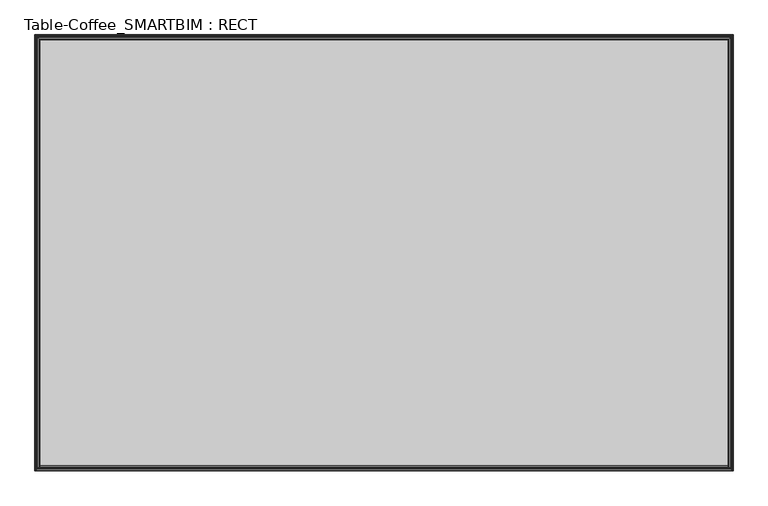
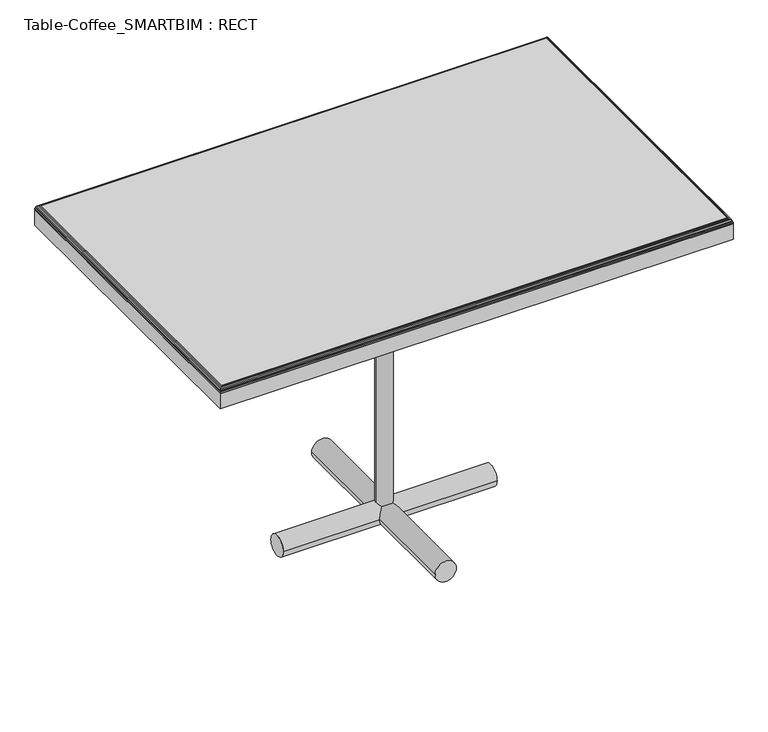
"""IFC4 building model written with IfcOpenShell, lengths in millimetres: furniture geometry, Table-Coffee_SMARTBIM : RECT."""

import ifcopenshell
import ifcopenshell.guid

model = None  # the IFC model being written
_history = None  # IfcOwnerHistory: only IFC2X3 demands one
_inside = {}  # id of a spatial element -> (the spatial element, [elements in it])
_under = {}  # id of a project, library or spatial element -> (it, [spatial elements below it])
_declared = {}  # id of a project -> (the project, [libraries it declares])
_typed = {}  # id of a type object -> (the type object, [elements of that type])
_made_of = {}  # id of a material, layer set ... -> (it, [elements and type objects made of it])


def new_model(schema):
    """Start an empty IFC model of exactly this schema.

    Asked for "IFC4X3", IfcOpenShell would pick the latest addendum, in which some entities
    have other attributes; the version numbers below select the first issue.
    IFC2X3 requires an IfcOwnerHistory on every rooted entity: one is made here for all.
    """
    global model, _history
    if schema == "IFC4X3":
        model = ifcopenshell.file(schema_version=(4, 3, 0, 0))
    else:
        model = ifcopenshell.file(schema=schema)
    _inside.clear()
    _under.clear()
    _declared.clear()
    _typed.clear()
    _made_of.clear()
    _history = None
    if model.schema == "IFC2X3":
        org = make("IfcOrganization", Name="unknown")
        user = make(
            "IfcPersonAndOrganization",
            ThePerson=make("IfcPerson", FamilyName="unknown"),
            TheOrganization=org,
        )
        app = make(
            "IfcApplication",
            ApplicationDeveloper=org,
            Version="unknown",
            ApplicationFullName="unknown",
            ApplicationIdentifier="unknown",
        )
        _history = make(
            "IfcOwnerHistory",
            OwningUser=user,
            OwningApplication=app,
            ChangeAction="ADDED",
            CreationDate=0,
        )
    return model


def make(cls, **values):
    """One entity of the class cls with the attributes given. An attribute that is None is left unset."""
    return model.create_entity(
        cls, **{name: value for name, value in values.items() if value is not None}
    )


def rooted(cls, **values):
    """An entity with a GlobalId (a new one), such as an element, a storey or a relation."""
    return make(cls, GlobalId=ifcopenshell.guid.new(), OwnerHistory=_history, **values)


def si_unit(unit_type, name, prefix=None):
    """IfcSIUnit, for example si_unit("LENGTHUNIT", "METRE", prefix="MILLI")."""
    return make("IfcSIUnit", UnitType=unit_type, Prefix=prefix, Name=name)


def assignment(units):
    """IfcUnitAssignment: the units of a project."""
    return None if units is None else make("IfcUnitAssignment", Units=units)


def point(xyz):
    """IfcCartesianPoint."""
    return None if xyz is None else make("IfcCartesianPoint", Coordinates=xyz)


def direction(xyz):
    """IfcDirection."""
    return None if xyz is None else make("IfcDirection", DirectionRatios=xyz)


def frame(location, z_axis=None, x_axis=None):
    """IfcAxis2Placement3D, a coordinate frame: its origin and axes. An axis left out is left unset."""
    return make(
        "IfcAxis2Placement3D",
        Location=point(location),
        Axis=direction(z_axis),
        RefDirection=direction(x_axis),
    )


def frame_2d(location, x_axis=None):
    """IfcAxis2Placement2D, a coordinate frame in the plane: its origin and x axis."""
    return make(
        "IfcAxis2Placement2D", Location=point(location), RefDirection=direction(x_axis)
    )


def origin():
    """The frame at (0, 0, 0) with its axes left unset."""
    return frame((0.0, 0.0, 0.0))


def origin_2d():
    """The frame at (0, 0) in the plane with its x axis left unset."""
    return frame_2d((0.0, 0.0))


def place(relative_to, where):
    """IfcLocalPlacement: puts the frame where relative to a parent placement (None: the world)."""
    return make(
        "IfcLocalPlacement", PlacementRelTo=relative_to, RelativePlacement=where
    )


def context(
    kind, dimensions, precision=None, world=None, true_north=None, identifier=None
):
    """IfcGeometricRepresentationContext, for example the 3D "Model" context."""
    return make(
        "IfcGeometricRepresentationContext",
        ContextIdentifier=identifier,
        ContextType=kind,
        CoordinateSpaceDimension=dimensions,
        Precision=precision,
        WorldCoordinateSystem=world,
        TrueNorth=true_north,
    )


def project(units=None, contexts=None):
    """IfcProject with its units and contexts."""
    return rooted(
        "IfcProject",
        Name="project",
        RepresentationContexts=contexts,
        UnitsInContext=assignment(units),
    )


def spatial(cls, under=None, at=None, **own):
    """A site, building, storey or space (cls), placed at a placement, below another one or the project."""
    s = rooted(cls, ObjectPlacement=at, **own)
    if under is not None:
        _under.setdefault(under.id(), (under, []))[1].append(s)
    return s


def polyline(points):
    """IfcPolyline through the points."""
    return make("IfcPolyline", Points=[point(p) for p in points])


def circle_curve(where, radius):
    """IfcCircle in the frame where."""
    return make("IfcCircle", Position=where, Radius=radius)


def ellipse_curve(where, semi_axis1, semi_axis2):
    """IfcEllipse in the frame where."""
    return make(
        "IfcEllipse", Position=where, SemiAxis1=semi_axis1, SemiAxis2=semi_axis2
    )


def trimmed(basis, trim1, trim2, sense, master):
    """IfcTrimmedCurve: the piece of a basis curve between two trims."""
    return make(
        "IfcTrimmedCurve",
        BasisCurve=basis,
        Trim1=trim1,
        Trim2=trim2,
        SenseAgreement=sense,
        MasterRepresentation=master,
    )


def segment(curve, same_sense, transition):
    """IfcCompositeCurveSegment."""
    return make(
        "IfcCompositeCurveSegment",
        Transition=transition,
        SameSense=same_sense,
        ParentCurve=curve,
    )


def composite_curve(segments, self_intersect=None):
    """IfcCompositeCurve: segments joined end to end."""
    return make("IfcCompositeCurve", Segments=segments, SelfIntersect=self_intersect)


def outline(outer, holes=None, kind="AREA"):
    """IfcArbitraryClosedProfileDef: a profile drawn as a closed curve; with holes, ...WithVoids."""
    if holes is None:
        return make("IfcArbitraryClosedProfileDef", ProfileType=kind, OuterCurve=outer)
    return make(
        "IfcArbitraryProfileDefWithVoids",
        ProfileType=kind,
        OuterCurve=outer,
        InnerCurves=holes,
    )


def extrude(swept, where, along, depth):
    """IfcExtrudedAreaSolid: the profile swept, set in the frame where, extruded along a direction by depth."""
    return make(
        "IfcExtrudedAreaSolid",
        SweptArea=swept,
        Position=where,
        ExtrudedDirection=direction(along),
        Depth=depth,
    )


def shape(context_of_items, identifier, shape_type, items):
    """IfcShapeRepresentation: the items that make up one representation, for example the "Body"."""
    return make(
        "IfcShapeRepresentation",
        ContextOfItems=context_of_items,
        RepresentationIdentifier=identifier,
        RepresentationType=shape_type,
        Items=items,
    )


def source(mapping_origin, context_of_items, identifier, shape_type, items):
    """IfcRepresentationMap: a shape defined once, which mapped items show again and again."""
    return make(
        "IfcRepresentationMap",
        MappingOrigin=mapping_origin,
        MappedRepresentation=shape(context_of_items, identifier, shape_type, items),
    )


def transform(
    local_origin,
    x_axis=None,
    y_axis=None,
    z_axis=None,
    scale=None,
    scale2=None,
    scale3=None,
    uniform=True,
):
    """IfcCartesianTransformationOperator3D, or its non-uniform kind. x_axis, y_axis, z_axis: its Axis1, 2, 3."""
    if uniform:
        return make(
            "IfcCartesianTransformationOperator3D",
            Axis1=direction(x_axis),
            Axis2=direction(y_axis),
            LocalOrigin=point(local_origin),
            Scale=scale,
            Axis3=direction(z_axis),
        )
    return make(
        "IfcCartesianTransformationOperator3DnonUniform",
        Axis1=direction(x_axis),
        Axis2=direction(y_axis),
        LocalOrigin=point(local_origin),
        Scale=scale,
        Axis3=direction(z_axis),
        Scale2=scale2,
        Scale3=scale3,
    )


def mapped(mapping_source, mapping_target):
    """IfcMappedItem: shows the shape of a source again, moved by a transform."""
    return make(
        "IfcMappedItem", MappingSource=mapping_source, MappingTarget=mapping_target
    )


def made_of(thing, what):
    """Note that an element or type object is made of a material, layer set ...; save() writes the relation."""
    if what is not None:
        _made_of.setdefault(what.id(), (what, []))[1].append(thing)
    return thing


def element(
    cls,
    number,
    at=None,
    inside=None,
    cuts=None,
    type_object=None,
    material=None,
    context=None,
    identifier="Body",
    shape_type=None,
    held_by="IfcProductDefinitionShape",
    body=None,
    shapes=None,
    **own,
):
    """One element of the class cls, such as IfcWall. Its Tag is "e" and its number.

    at: its placement. inside: the storey or other place that contains it. cuts: it is an
    opening in that element (IfcRelVoidsElement). A single representation is given by context,
    identifier, shape_type and body (its items); several are given by shapes. held_by: the class
    of the entity that holds the representations. save() writes the other relations.
    """
    e = rooted(cls, Tag="e%d" % number, ObjectPlacement=at, **own)
    if body is not None:
        shapes = [shape(context, identifier, shape_type, body)]
    if shapes is not None:
        e.Representation = make(held_by, Representations=shapes)
    if inside is not None:
        _inside.setdefault(inside.id(), (inside, []))[1].append(e)
    if cuts is not None:
        rooted(
            "IfcRelVoidsElement", RelatingBuildingElement=cuts, RelatedOpeningElement=e
        )
    if type_object is not None:
        _typed.setdefault(type_object.id(), (type_object, []))[1].append(e)
    return made_of(e, material)


def aggregate(whole, parts):
    """IfcRelAggregates: a whole, such as a stair, and the parts it consists of."""
    return rooted("IfcRelAggregates", RelatingObject=whole, RelatedObjects=parts)


def save(model, path):
    """Write the relations noted so far, then the file.

    IfcRelAggregates (storeys below a building ...), IfcRelContainedInSpatialStructure (elements
    in a storey), IfcRelDefinesByType, IfcRelAssociatesMaterial and IfcRelDeclares: one each for
    every whole, place, type object, material and project.
    """
    for whole, parts in _under.values():
        aggregate(whole, parts)
    for where, things in _inside.values():
        rooted(
            "IfcRelContainedInSpatialStructure",
            RelatedElements=things,
            RelatingStructure=where,
        )
    for kind, things in _typed.values():
        rooted("IfcRelDefinesByType", RelatedObjects=things, RelatingType=kind)
    for what, things in _made_of.values():
        rooted("IfcRelAssociatesMaterial", RelatedObjects=things, RelatingMaterial=what)
    for by, libraries in _declared.values():
        rooted("IfcRelDeclares", RelatingContext=by, RelatedDefinitions=libraries)
    model.write(path)


def plane_surface(at):
    """IfcPlane: the flat surface through the origin of the frame at, square to its z axis."""
    return make("IfcPlane", Position=at)


def cylinder_surface(at, radius):
    """IfcCylindricalSurface: all points at the distance radius from the z axis of the frame at."""
    return make("IfcCylindricalSurface", Position=at, Radius=radius)


def advanced_brep(points, edges, surfaces, faces):
    """IfcAdvancedBrep: a solid bounded by faces that lie on surfaces and meet in shared edges.

    An edge is (start, end): straight between two places in points (the first is 0);
    or (start, end, curve); or (start, end, curve, False) where it runs against its curve.
    A face is (place in surfaces, loops), or (place, loops, False) where it looks against
    its surface's normal. A loop lists edges by number (the first is 1), with a minus sign
    where the edge is run from its end to its start. The first loop is the outer one.
    """
    corners = [point(p) for p in points]
    vertices = [make("IfcVertexPoint", VertexGeometry=c) for c in corners]
    made = []
    for start, end, *more in edges:
        made.append(
            make(
                "IfcEdgeCurve",
                EdgeStart=vertices[start],
                EdgeEnd=vertices[end],
                EdgeGeometry=more[0] if more else make("IfcPolyline", Points=[corners[start], corners[end]]),
                SameSense=more[1] if len(more) > 1 else True,
            )
        )
    hull = []
    for where, loops, *sense in faces:
        bounds = []
        for j, loop in enumerate(loops):
            ring = [make("IfcOrientedEdge", EdgeElement=made[abs(k) - 1], Orientation=k > 0) for k in loop]
            bounds.append(
                make(
                    "IfcFaceOuterBound" if j == 0 else "IfcFaceBound",
                    Bound=make("IfcEdgeLoop", EdgeList=ring),
                    Orientation=True,
                )
            )
        hull.append(make("IfcAdvancedFace", Bounds=bounds, FaceSurface=surfaces[where], SameSense=sense[0] if sense else True))
    return make("IfcAdvancedBrep", Outer=make("IfcClosedShell", CfsFaces=hull))


def table_coffee_smartbim_rect_06f34b69(model_context):
    return source(origin(), model_context, "Body", "SolidModel", [
        extrude(outline(composite_curve([segment(trimmed(circle_curve(frame_2d((0.0, 25.4)), 25.4), [point((-25.4, 25.4))], [point((25.4, 25.4))], False, "CARTESIAN"), True, "CONTINUOUS"), segment(trimmed(circle_curve(frame_2d((0.0, 25.4)), 25.4), [point((25.4, 25.4))], [point((-25.4, 25.4))], False, "CARTESIAN"), True, "CONTINUOUS")], self_intersect=False)), frame((-254.0, 0.0, 0.0), z_axis=(1.0, 0.0, 0.0), x_axis=(0.0, 1.0, 0.0)), (0.0, 0.0, 1.0), 508.0),
        extrude(outline(composite_curve([segment(trimmed(circle_curve(frame_2d((25.4, 0.0)), 25.4), [point((25.4, -25.4))], [point((25.4, 25.4))], False, "CARTESIAN"), True, "CONTINUOUS"), segment(trimmed(circle_curve(frame_2d((25.4, 0.0)), 25.4), [point((25.4, 25.4))], [point((25.4, -25.4))], False, "CARTESIAN"), True, "CONTINUOUS")], self_intersect=False)), frame((0.0, -254.0, 0.0), z_axis=(0.0, 1.0, 0.0), x_axis=(0.0, 0.0, 1.0)), (0.0, 0.0, 1.0), 508.0),
        extrude(outline(polyline([(609.6, -381.0), (-609.6, -381.0), (-609.6, 381.0), (609.6, 381.0), (609.6, -381.0)])), frame((0.0, 0.0, 723.9), z_axis=(0.0, 0.0, 1.0), x_axis=(1.0, 0.0, 0.0)), (0.0, 0.0, 1.0), 38.1),
        advanced_brep(
        [(-600.1998654, 371.5998654, 774.7), (-600.1998654, -371.5998654, 774.7), (600.1998654, -371.5998654, 774.7), (600.1998654, 371.5998654, 774.7), (609.6, -381.0, 762.0), (-609.6, -381.0, 762.0), (-609.6, 381.0, 762.0), (609.6, 381.0, 762.0), (609.6, -381.0, 765.2998654), (-609.6, -381.0, 765.2998654), (-609.6, 381.0, 765.2998654), (609.6, 381.0, 765.2998654), (-609.2372483, -380.6372483, 767.8860287), (-609.2372483, 380.6372483, 767.8860287), (-602.3616212, -373.7616212, 774.4480533), (-602.3616212, 373.7616212, 774.4480533), (-604.3639185, 375.7639185, 773.7273912), (-604.3639185, -375.7639185, 773.7273912), (-606.4885738, 377.8885738, 772.2866155), (-606.4885738, -377.8885738, 772.2866155), (-608.5102962, 379.9102962, 769.692959), (-608.5102962, -379.9102962, 769.692959), (609.2372483, 380.6372483, 767.8860287), (602.3616212, 373.7616212, 774.4480533), (604.3639185, 375.7639185, 773.7273912), (606.4885738, 377.8885738, 772.2866155), (608.5102962, 379.9102962, 769.692959), (609.2372483, -380.6372483, 767.8860287), (602.3616212, -373.7616212, 774.4480533), (604.3639185, -375.7639185, 773.7273912), (606.4885738, -377.8885738, 772.2866155), (608.5102962, -379.9102962, 769.692959)],
        [
            (0, 1),
            (1, 2),
            (2, 3),
            (3, 0),
            (4, 5),
            (5, 6),
            (6, 7),
            (7, 4),
            (4, 8),
            (8, 9),
            (9, 5),
            (9, 10),
            (10, 6),
            (10, 11),
            (11, 7),
            (11, 8),
            (9, 12, ellipse_curve(frame((-600.1998654, -371.5998654, 765.2998654), z_axis=(-0.7071067811865475, 0.7071067811865475, 0.0), x_axis=(0.7071067811865474, 0.7071067811865476, 0.0)), 13.2937978, 9.4001346)),
            (12, 13),
            (13, 10, ellipse_curve(frame((-600.1998654, 371.5998654, 765.2998654), z_axis=(-0.7071067811865475, -0.7071067811865475, 0.0), x_axis=(-0.7071067811865474, 0.7071067811865476, 0.0)), 13.2937978, 9.4001346)),
            (14, 1, ellipse_curve(frame((-600.1998654, -371.5998654, 765.2998654), z_axis=(-0.7071067811865475, 0.7071067811865475, 0.0), x_axis=(0.7071067811865474, 0.7071067811865476, 0.0)), 13.2937978, 9.4001346)),
            (0, 15, ellipse_curve(frame((-600.1998654, 371.5998654, 765.2998654), z_axis=(-0.7071067811865475, -0.7071067811865475, 0.0), x_axis=(-0.7071067811865474, 0.7071067811865476, 0.0)), 13.2937978, 9.4001346)),
            (15, 14),
            (15, 16, ellipse_curve(frame((-600.1998654, 371.5998654, 765.2998654), z_axis=(-0.7071067811865475, -0.7071067811865475, 0.0), x_axis=(-0.7071067811865474, 0.7071067811865476, 0.0)), 13.2937978, 9.4001346)),
            (16, 17),
            (17, 14, ellipse_curve(frame((-600.1998654, -371.5998654, 765.2998654), z_axis=(-0.7071067811865475, 0.7071067811865475, 0.0), x_axis=(0.7071067811865474, 0.7071067811865476, 0.0)), 13.2937978, 9.4001346)),
            (16, 18, ellipse_curve(frame((-600.1998654, 371.5998654, 765.2998654), z_axis=(-0.7071067811865475, -0.7071067811865475, 0.0), x_axis=(-0.7071067811865474, 0.7071067811865476, 0.0)), 13.2937978, 9.4001346)),
            (18, 19),
            (19, 17, ellipse_curve(frame((-600.1998654, -371.5998654, 765.2998654), z_axis=(-0.7071067811865475, 0.7071067811865475, 0.0), x_axis=(0.7071067811865474, 0.7071067811865476, 0.0)), 13.2937978, 9.4001346)),
            (18, 20, ellipse_curve(frame((-600.1998654, 371.5998654, 765.2998654), z_axis=(-0.7071067811865475, -0.7071067811865475, 0.0), x_axis=(-0.7071067811865474, 0.7071067811865476, 0.0)), 13.2937978, 9.4001346)),
            (20, 21),
            (21, 19, ellipse_curve(frame((-600.1998654, -371.5998654, 765.2998654), z_axis=(-0.7071067811865475, 0.7071067811865475, 0.0), x_axis=(0.7071067811865474, 0.7071067811865476, 0.0)), 13.2937978, 9.4001346)),
            (12, 21, ellipse_curve(frame((-600.1998654, -371.5998654, 765.2998654), z_axis=(-0.7071067811865475, 0.7071067811865475, 0.0), x_axis=(0.7071067811865474, 0.7071067811865476, 0.0)), 13.2937978, 9.4001346)),
            (20, 13, ellipse_curve(frame((-600.1998654, 371.5998654, 765.2998654), z_axis=(-0.7071067811865475, -0.7071067811865475, 0.0), x_axis=(-0.7071067811865474, 0.7071067811865476, 0.0)), 13.2937978, 9.4001346)),
            (13, 22),
            (22, 11, ellipse_curve(frame((600.1998654, 371.5998654, 765.2998654), z_axis=(-0.7071067811865475, 0.7071067811865475, 0.0), x_axis=(0.7071067811865476, 0.7071067811865474, 0.0)), 13.2937978, 9.4001346)),
            (3, 23, ellipse_curve(frame((600.1998654, 371.5998654, 765.2998654), z_axis=(-0.7071067811865475, 0.7071067811865475, 0.0), x_axis=(0.7071067811865476, 0.7071067811865474, 0.0)), 13.2937978, 9.4001346)),
            (23, 15),
            (23, 24, ellipse_curve(frame((600.1998654, 371.5998654, 765.2998654), z_axis=(-0.7071067811865475, 0.7071067811865475, 0.0), x_axis=(0.7071067811865476, 0.7071067811865474, 0.0)), 13.2937978, 9.4001346)),
            (24, 16),
            (24, 25, ellipse_curve(frame((600.1998654, 371.5998654, 765.2998654), z_axis=(-0.7071067811865475, 0.7071067811865475, 0.0), x_axis=(0.7071067811865476, 0.7071067811865474, 0.0)), 13.2937978, 9.4001346)),
            (25, 18),
            (25, 26, ellipse_curve(frame((600.1998654, 371.5998654, 765.2998654), z_axis=(-0.7071067811865475, 0.7071067811865475, 0.0), x_axis=(0.7071067811865476, 0.7071067811865474, 0.0)), 13.2937978, 9.4001346)),
            (26, 20),
            (26, 22, ellipse_curve(frame((600.1998654, 371.5998654, 765.2998654), z_axis=(-0.7071067811865475, 0.7071067811865475, 0.0), x_axis=(0.7071067811865476, 0.7071067811865474, 0.0)), 13.2937978, 9.4001346)),
            (22, 27),
            (27, 8, ellipse_curve(frame((600.1998654, -371.5998654, 765.2998654), z_axis=(0.7071067811865475, 0.7071067811865475, 0.0), x_axis=(0.7071067811865474, -0.7071067811865476, 0.0)), 13.2937978, 9.4001346)),
            (2, 28, ellipse_curve(frame((600.1998654, -371.5998654, 765.2998654), z_axis=(0.7071067811865475, 0.7071067811865475, 0.0), x_axis=(0.7071067811865474, -0.7071067811865476, 0.0)), 13.2937978, 9.4001346)),
            (28, 23),
            (28, 29, ellipse_curve(frame((600.1998654, -371.5998654, 765.2998654), z_axis=(0.7071067811865475, 0.7071067811865475, 0.0), x_axis=(0.7071067811865474, -0.7071067811865476, 0.0)), 13.2937978, 9.4001346)),
            (29, 24),
            (29, 30, ellipse_curve(frame((600.1998654, -371.5998654, 765.2998654), z_axis=(0.7071067811865475, 0.7071067811865475, 0.0), x_axis=(0.7071067811865474, -0.7071067811865476, 0.0)), 13.2937978, 9.4001346)),
            (30, 25),
            (30, 31, ellipse_curve(frame((600.1998654, -371.5998654, 765.2998654), z_axis=(0.7071067811865475, 0.7071067811865475, 0.0), x_axis=(0.7071067811865474, -0.7071067811865476, 0.0)), 13.2937978, 9.4001346)),
            (31, 26),
            (31, 27, ellipse_curve(frame((600.1998654, -371.5998654, 765.2998654), z_axis=(0.7071067811865475, 0.7071067811865475, 0.0), x_axis=(0.7071067811865474, -0.7071067811865476, 0.0)), 13.2937978, 9.4001346)),
            (27, 12),
            (14, 28),
            (17, 29),
            (19, 30),
            (21, 31),
        ],
        [
            plane_surface(frame((-609.6, -381.0, 774.7), z_axis=(0.0, 0.0, 1.0), x_axis=(-1.0, 0.0, 0.0))),
            plane_surface(frame((-609.6, -381.0, 762.0), z_axis=(0.0, 0.0, -1.0), x_axis=(1.0, 0.0, 0.0))),
            plane_surface(frame((609.6, -381.0, 774.7), z_axis=(0.0, -1.0, 0.0), x_axis=(0.0, 0.0, -1.0))),
            plane_surface(frame((-609.6, -381.0, 774.7), z_axis=(-1.0, 0.0, 0.0), x_axis=(0.0, 0.0, -1.0))),
            plane_surface(frame((-609.6, 381.0, 774.7), z_axis=(0.0, 1.0, 0.0), x_axis=(0.0, 0.0, -1.0))),
            plane_surface(frame((609.6, 381.0, 774.7), z_axis=(1.0, 0.0, 0.0), x_axis=(0.0, 0.0, -1.0))),
            cylinder_surface(frame((-600.1998654, -381.0, 765.2998654), z_axis=(0.0, 1.0, 0.0), x_axis=(1.0, 0.0, 0.0)), 9.4001346),
            cylinder_surface(frame((-609.6, 371.5998654, 765.2998654), z_axis=(1.0, 0.0, 0.0), x_axis=(0.0, -1.0, 0.0)), 9.4001346),
            cylinder_surface(frame((600.1998654, 381.0, 765.2998654), z_axis=(0.0, -1.0, 0.0), x_axis=(-1.0, 0.0, 0.0)), 9.4001346),
            cylinder_surface(frame((609.6, -371.5998654, 765.2998654), z_axis=(-1.0, 0.0, 0.0), x_axis=(0.0, 1.0, 0.0)), 9.4001346),
        ],
        [
            (0, [[1, 2, 3, 4]]),
            (1, [[5, 6, 7, 8]]),
            (2, [[9, 10, 11, -5]]),
            (3, [[-11, 12, 13, -6]]),
            (4, [[-13, 14, 15, -7]]),
            (5, [[-15, 16, -9, -8]]),
            (6, [[-12, 17, 18, 19]]),
            (6, [[20, -1, 21, 22]]),
            (6, [[23, 24, 25, -22]]),
            (6, [[26, 27, 28, -24]]),
            (6, [[29, 30, 31, -27]]),
            (6, [[32, -30, 33, -18]]),
            (7, [[34, 35, -14, -19]]),
            (7, [[-4, 36, 37, -21]]),
            (7, [[-37, 38, 39, -23]]),
            (7, [[-39, 40, 41, -26]]),
            (7, [[-41, 42, 43, -29]]),
            (7, [[-43, 44, -34, -33]]),
            (8, [[45, 46, -16, -35]]),
            (8, [[-3, 47, 48, -36]]),
            (8, [[-48, 49, 50, -38]]),
            (8, [[-50, 51, 52, -40]]),
            (8, [[-52, 53, 54, -42]]),
            (8, [[-54, 55, -45, -44]]),
            (9, [[-10, -46, 56, -17]]),
            (9, [[57, -47, -2, -20]]),
            (9, [[58, -49, -57, -25]]),
            (9, [[59, -51, -58, -28]]),
            (9, [[60, -53, -59, -31]]),
            (9, [[-56, -55, -60, -32]]),
        ],
    ),
        extrude(outline(polyline([(76.2, -76.2), (-76.2, -76.2), (-76.2, 76.2), (76.2, 76.2), (76.2, -76.2)])), frame((0.0, 0.0, 755.65), z_axis=(0.0, 0.0, 1.0), x_axis=(1.0, 0.0, 0.0)), (0.0, 0.0, 1.0), 6.35),
        extrude(outline(composite_curve([segment(trimmed(circle_curve(origin_2d(), 19.05), [point((-19.05, 0.0))], [point((19.05, 0.0))], False, "CARTESIAN"), True, "CONTINUOUS"), segment(trimmed(circle_curve(origin_2d(), 19.05), [point((19.05, 0.0))], [point((-19.05, 0.0))], False, "CARTESIAN"), True, "CONTINUOUS")], self_intersect=False)), frame((0.0, 0.0, 24.2070278), z_axis=(0.0, 0.0, 1.0), x_axis=(1.0, 0.0, 0.0)), (0.0, 0.0, 1.0), 731.4429722),
    ])


if __name__ == "__main__":
    model = new_model("IFC4")
    model_context = context("Model", 3, world=origin())
    ifc_project = project(units=[si_unit("LENGTHUNIT", "METRE", prefix="MILLI")], contexts=[model_context])
    site = spatial("IfcSite", under=ifc_project)
    building = spatial("IfcBuilding", under=site)
    placement = place(None, origin())
    table_coffee_smartbim_rect_shape = table_coffee_smartbim_rect_06f34b69(model_context)
    element("IfcFurniture", 1, ObjectType="Table-Coffee_SMARTBIM : RECT", at=placement, inside=building, context=model_context, shape_type="MappedRepresentation", body=[
        mapped(table_coffee_smartbim_rect_shape, transform((0.0, 0.0, 0.0), x_axis=(1.0, 0.0, 0.0), y_axis=(0.0, 1.0, 0.0), z_axis=(0.0, 0.0, 1.0))),
    ])
    save(model, "model.ifc")

# Revit data of these elements
# Project information
#   Project Issue Date = "08/08/2019"
#   Project Status = "Project Status"
#   Client Name = "Owner"
#   Project Address = "SOMERS, WI"
#   Project Name = "OAKFIRE 2.0"
#   Project Number = "Project Number"
# Type "Table-Coffee_SMARTBIM : RECT"
#   Subcategory = "Table\r\n"
#   SmartBIM Object Created By = "SMARTBIM, LLC"
#   Manufacturer = "SMARTBIM"
#   Assembly Code = "E2020200"
#   95 CSI = "12500"
#   04 CSI = "12 50 00"
#   table cloth = 0' - 1 1/2"
#   Width = 4' - 0"
#   SmartBIM Object Version = 3
#   Height = 2' - 6"
#   Depth = 2' - 6"
#   Default Elevation = 4' - 0"
#   white cloth_parameter = WOOD-OAKFIRE
#   Table Unit = MET
#   Glide = none
#   Glass = none
# Element 1 (IfcFurniture, "Table-Coffee_SMARTBIM : RECT")
#   Materials on its faces: "WOOD-OAKFIRE", "MET"
# Materials
#   "WOOD-OAKFIRE": class "Wood", colour RGB 198 202 183, transparency 0, Description = "Generic wood", Cost = 0
#   "MET": class "Metal", colour RGB 189 187 185, transparency 0
